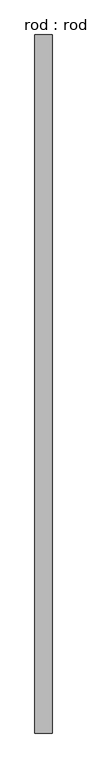
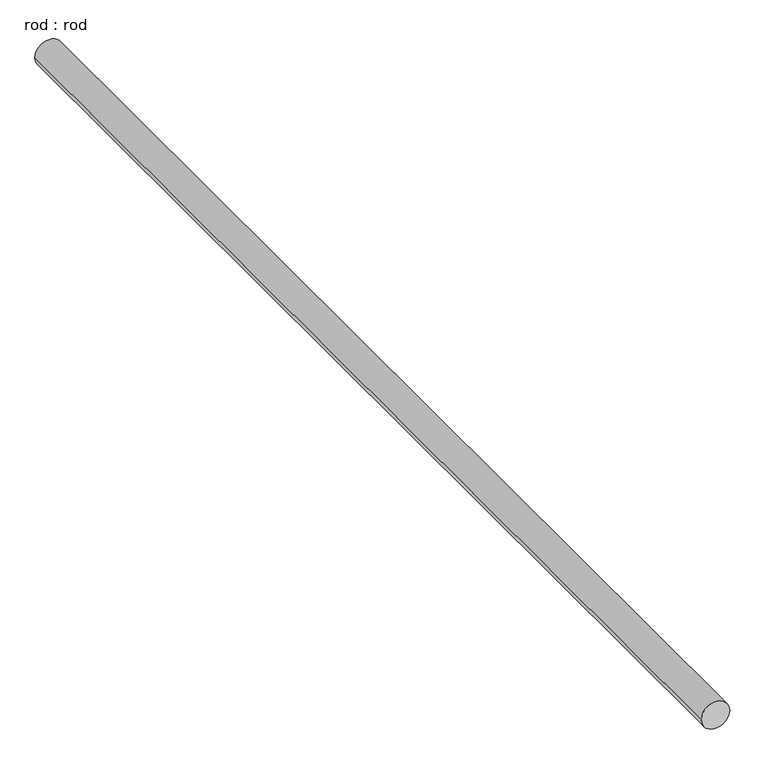
"""IFC4 building model written with IfcOpenShell, lengths in millimetres: proxy geometry, rod : rod."""

from ifc_helpers import new_model, si_unit, point, frame, frame_2d, origin, place, context, project, spatial, circle_curve, trimmed, segment, composite_curve, outline, extrude, source, transform, mapped, element, save


def rod_rod_8513d977(model_context):
    return source(origin(), model_context, "Body", "SweptSolid", [
        extrude(outline(composite_curve([segment(trimmed(circle_curve(frame_2d((0.0108462, 0.0)), 200.0), [point((0.0108462, 200.0))], [point((0.0108462, -200.0))], False, "CARTESIAN"), True, "CONTINUOUS"), segment(trimmed(circle_curve(frame_2d((0.0108462, 0.0)), 200.0), [point((0.0108462, -200.0))], [point((0.0108462, 200.0))], False, "CARTESIAN"), True, "CONTINUOUS")], self_intersect=False)), frame((0.0, -4050.1285275, 0.0), z_axis=(0.0, 1.0, 0.0), x_axis=(0.0, 0.0, 1.0)), (0.0, 0.0, 1.0), 16285.7142857),
    ])


if __name__ == "__main__":
    model = new_model("IFC4")
    model_context = context("Model", 3, world=origin())
    ifc_project = project(units=[si_unit("LENGTHUNIT", "METRE", prefix="MILLI")], contexts=[model_context])
    site = spatial("IfcSite", under=ifc_project)
    building = spatial("IfcBuilding", under=site)
    placement = place(None, origin())
    rod_rod_shape = rod_rod_8513d977(model_context)
    element("IfcBuildingElementProxy", 1, Name="rod : rod", ObjectType="rod : rod", at=placement, inside=building, context=model_context, shape_type="MappedRepresentation", body=[
        mapped(rod_rod_shape, transform((0.0, 0.0, 0.0), x_axis=(1.0, 0.0, 0.0), y_axis=(0.0, 1.0, 0.0), z_axis=(0.0, 0.0, 1.0))),
    ])
    save(model, "model.ifc")

# Revit data of these elements
# Type "rod : rod"
#   Default Elevation = 0
